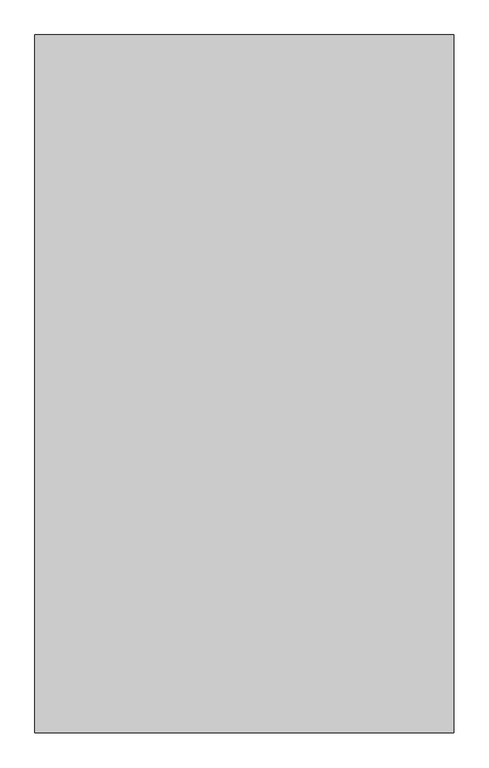
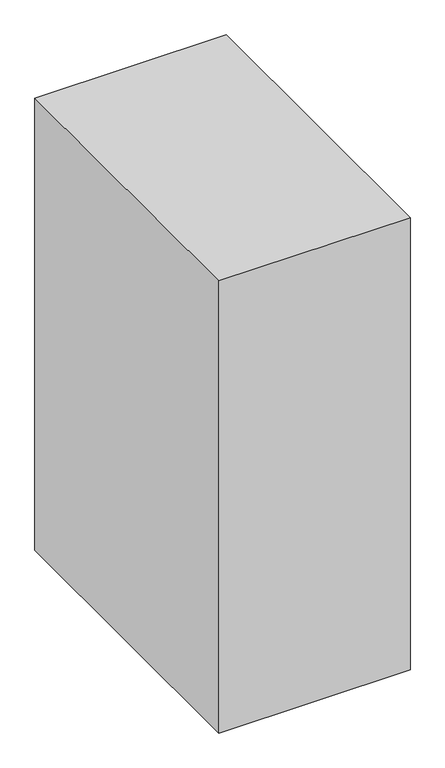
"""IFC4 building model written with IfcOpenShell, lengths in millimetres: proxy geometry, Space Planning Box_hec : Space Planning Box_hec."""

import ifcopenshell
import ifcopenshell.guid

model = None  # the IFC model being written
_history = None  # IfcOwnerHistory: only IFC2X3 demands one
_inside = {}  # id of a spatial element -> (the spatial element, [elements in it])
_under = {}  # id of a project, library or spatial element -> (it, [spatial elements below it])
_declared = {}  # id of a project -> (the project, [libraries it declares])
_typed = {}  # id of a type object -> (the type object, [elements of that type])
_made_of = {}  # id of a material, layer set ... -> (it, [elements and type objects made of it])


def new_model(schema):
    """Start an empty IFC model of exactly this schema.

    Asked for "IFC4X3", IfcOpenShell would pick the latest addendum, in which some entities
    have other attributes; the version numbers below select the first issue.
    IFC2X3 requires an IfcOwnerHistory on every rooted entity: one is made here for all.
    """
    global model, _history
    if schema == "IFC4X3":
        model = ifcopenshell.file(schema_version=(4, 3, 0, 0))
    else:
        model = ifcopenshell.file(schema=schema)
    _inside.clear()
    _under.clear()
    _declared.clear()
    _typed.clear()
    _made_of.clear()
    _history = None
    if model.schema == "IFC2X3":
        org = make("IfcOrganization", Name="unknown")
        user = make(
            "IfcPersonAndOrganization",
            ThePerson=make("IfcPerson", FamilyName="unknown"),
            TheOrganization=org,
        )
        app = make(
            "IfcApplication",
            ApplicationDeveloper=org,
            Version="unknown",
            ApplicationFullName="unknown",
            ApplicationIdentifier="unknown",
        )
        _history = make(
            "IfcOwnerHistory",
            OwningUser=user,
            OwningApplication=app,
            ChangeAction="ADDED",
            CreationDate=0,
        )
    return model


def make(cls, **values):
    """One entity of the class cls with the attributes given. An attribute that is None is left unset."""
    return model.create_entity(
        cls, **{name: value for name, value in values.items() if value is not None}
    )


def rooted(cls, **values):
    """An entity with a GlobalId (a new one), such as an element, a storey or a relation."""
    return make(cls, GlobalId=ifcopenshell.guid.new(), OwnerHistory=_history, **values)


def si_unit(unit_type, name, prefix=None):
    """IfcSIUnit, for example si_unit("LENGTHUNIT", "METRE", prefix="MILLI")."""
    return make("IfcSIUnit", UnitType=unit_type, Prefix=prefix, Name=name)


def assignment(units):
    """IfcUnitAssignment: the units of a project."""
    return None if units is None else make("IfcUnitAssignment", Units=units)


def point(xyz):
    """IfcCartesianPoint."""
    return None if xyz is None else make("IfcCartesianPoint", Coordinates=xyz)


def direction(xyz):
    """IfcDirection."""
    return None if xyz is None else make("IfcDirection", DirectionRatios=xyz)


def frame(location, z_axis=None, x_axis=None):
    """IfcAxis2Placement3D, a coordinate frame: its origin and axes. An axis left out is left unset."""
    return make(
        "IfcAxis2Placement3D",
        Location=point(location),
        Axis=direction(z_axis),
        RefDirection=direction(x_axis),
    )


def origin():
    """The frame at (0, 0, 0) with its axes left unset."""
    return frame((0.0, 0.0, 0.0))


def origin_with_axes():
    """The frame at (0, 0, 0) with the z axis (0, 0, 1) and the x axis (1, 0, 0) written out."""
    return frame((0.0, 0.0, 0.0), z_axis=(0.0, 0.0, 1.0), x_axis=(1.0, 0.0, 0.0))


def place(relative_to, where):
    """IfcLocalPlacement: puts the frame where relative to a parent placement (None: the world)."""
    return make(
        "IfcLocalPlacement", PlacementRelTo=relative_to, RelativePlacement=where
    )


def context(
    kind, dimensions, precision=None, world=None, true_north=None, identifier=None
):
    """IfcGeometricRepresentationContext, for example the 3D "Model" context."""
    return make(
        "IfcGeometricRepresentationContext",
        ContextIdentifier=identifier,
        ContextType=kind,
        CoordinateSpaceDimension=dimensions,
        Precision=precision,
        WorldCoordinateSystem=world,
        TrueNorth=true_north,
    )


def project(units=None, contexts=None):
    """IfcProject with its units and contexts."""
    return rooted(
        "IfcProject",
        Name="project",
        RepresentationContexts=contexts,
        UnitsInContext=assignment(units),
    )


def spatial(cls, under=None, at=None, **own):
    """A site, building, storey or space (cls), placed at a placement, below another one or the project."""
    s = rooted(cls, ObjectPlacement=at, **own)
    if under is not None:
        _under.setdefault(under.id(), (under, []))[1].append(s)
    return s


def polyline(points):
    """IfcPolyline through the points."""
    return make("IfcPolyline", Points=[point(p) for p in points])


def outline(outer, holes=None, kind="AREA"):
    """IfcArbitraryClosedProfileDef: a profile drawn as a closed curve; with holes, ...WithVoids."""
    if holes is None:
        return make("IfcArbitraryClosedProfileDef", ProfileType=kind, OuterCurve=outer)
    return make(
        "IfcArbitraryProfileDefWithVoids",
        ProfileType=kind,
        OuterCurve=outer,
        InnerCurves=holes,
    )


def extrude(swept, where, along, depth):
    """IfcExtrudedAreaSolid: the profile swept, set in the frame where, extruded along a direction by depth."""
    return make(
        "IfcExtrudedAreaSolid",
        SweptArea=swept,
        Position=where,
        ExtrudedDirection=direction(along),
        Depth=depth,
    )


def shape(context_of_items, identifier, shape_type, items):
    """IfcShapeRepresentation: the items that make up one representation, for example the "Body"."""
    return make(
        "IfcShapeRepresentation",
        ContextOfItems=context_of_items,
        RepresentationIdentifier=identifier,
        RepresentationType=shape_type,
        Items=items,
    )


def source(mapping_origin, context_of_items, identifier, shape_type, items):
    """IfcRepresentationMap: a shape defined once, which mapped items show again and again."""
    return make(
        "IfcRepresentationMap",
        MappingOrigin=mapping_origin,
        MappedRepresentation=shape(context_of_items, identifier, shape_type, items),
    )


def transform(
    local_origin,
    x_axis=None,
    y_axis=None,
    z_axis=None,
    scale=None,
    scale2=None,
    scale3=None,
    uniform=True,
):
    """IfcCartesianTransformationOperator3D, or its non-uniform kind. x_axis, y_axis, z_axis: its Axis1, 2, 3."""
    if uniform:
        return make(
            "IfcCartesianTransformationOperator3D",
            Axis1=direction(x_axis),
            Axis2=direction(y_axis),
            LocalOrigin=point(local_origin),
            Scale=scale,
            Axis3=direction(z_axis),
        )
    return make(
        "IfcCartesianTransformationOperator3DnonUniform",
        Axis1=direction(x_axis),
        Axis2=direction(y_axis),
        LocalOrigin=point(local_origin),
        Scale=scale,
        Axis3=direction(z_axis),
        Scale2=scale2,
        Scale3=scale3,
    )


def mapped(mapping_source, mapping_target):
    """IfcMappedItem: shows the shape of a source again, moved by a transform."""
    return make(
        "IfcMappedItem", MappingSource=mapping_source, MappingTarget=mapping_target
    )


def made_of(thing, what):
    """Note that an element or type object is made of a material, layer set ...; save() writes the relation."""
    if what is not None:
        _made_of.setdefault(what.id(), (what, []))[1].append(thing)
    return thing


def element(
    cls,
    number,
    at=None,
    inside=None,
    cuts=None,
    type_object=None,
    material=None,
    context=None,
    identifier="Body",
    shape_type=None,
    held_by="IfcProductDefinitionShape",
    body=None,
    shapes=None,
    **own,
):
    """One element of the class cls, such as IfcWall. Its Tag is "e" and its number.

    at: its placement. inside: the storey or other place that contains it. cuts: it is an
    opening in that element (IfcRelVoidsElement). A single representation is given by context,
    identifier, shape_type and body (its items); several are given by shapes. held_by: the class
    of the entity that holds the representations. save() writes the other relations.
    """
    e = rooted(cls, Tag="e%d" % number, ObjectPlacement=at, **own)
    if body is not None:
        shapes = [shape(context, identifier, shape_type, body)]
    if shapes is not None:
        e.Representation = make(held_by, Representations=shapes)
    if inside is not None:
        _inside.setdefault(inside.id(), (inside, []))[1].append(e)
    if cuts is not None:
        rooted(
            "IfcRelVoidsElement", RelatingBuildingElement=cuts, RelatedOpeningElement=e
        )
    if type_object is not None:
        _typed.setdefault(type_object.id(), (type_object, []))[1].append(e)
    return made_of(e, material)


def aggregate(whole, parts):
    """IfcRelAggregates: a whole, such as a stair, and the parts it consists of."""
    return rooted("IfcRelAggregates", RelatingObject=whole, RelatedObjects=parts)


def save(model, path):
    """Write the relations noted so far, then the file.

    IfcRelAggregates (storeys below a building ...), IfcRelContainedInSpatialStructure (elements
    in a storey), IfcRelDefinesByType, IfcRelAssociatesMaterial and IfcRelDeclares: one each for
    every whole, place, type object, material and project.
    """
    for whole, parts in _under.values():
        aggregate(whole, parts)
    for where, things in _inside.values():
        rooted(
            "IfcRelContainedInSpatialStructure",
            RelatedElements=things,
            RelatingStructure=where,
        )
    for kind, things in _typed.values():
        rooted("IfcRelDefinesByType", RelatedObjects=things, RelatingType=kind)
    for what, things in _made_of.values():
        rooted("IfcRelAssociatesMaterial", RelatedObjects=things, RelatingMaterial=what)
    for by, libraries in _declared.values():
        rooted("IfcRelDeclares", RelatingContext=by, RelatedDefinitions=libraries)
    model.write(path)


def generic_models_47b98be1(model_context):
    return source(origin(), model_context, "Body", "SweptSolid", [
        extrude(outline(polyline([(1200.0, 2000.0), (1200.0, -2000.0), (-1200.0, -2000.0), (-1200.0, 2000.0), (1200.0, 2000.0)])), origin_with_axes(), (0.0, 0.0, 1.0), 6000.0),
    ])


if __name__ == "__main__":
    model = new_model("IFC4")
    model_context = context("Model", 3, world=origin())
    ifc_project = project(units=[si_unit("LENGTHUNIT", "METRE", prefix="MILLI")], contexts=[model_context])
    site = spatial("IfcSite", under=ifc_project)
    building = spatial("IfcBuilding", under=site)
    placement = place(None, origin())
    generic_models_shape = generic_models_47b98be1(model_context)
    element("IfcBuildingElementProxy", 1, Name="Space Planning Box_hec : Space Planning Box_hec", ObjectType="Space Planning Box_hec : Space Planning Box_hec", at=placement, inside=building, context=model_context, shape_type="MappedRepresentation", body=[
        mapped(generic_models_shape, transform((0.0, 0.0, 0.0), x_axis=(1.0, 0.0, 0.0), y_axis=(0.0, 1.0, 0.0), z_axis=(0.0, 0.0, 1.0))),
    ])
    save(model, "model.ifc")

# Revit data of these elements
# Type "Space Planning Box_hec : Space Planning Box_hec"
#   Type Comments = "..."
#   Room Name [instance default] = "?"
#   Interior Finish [instance default] = ""
#   Exterior Finish [instance default] = ""
#   Department [instance default] = ""
#   Assembly Code = "..."
#   Width [instance default] = 1524 mm
#   Program Area [instance default] = 0 m²
#   Length [instance default] = 1524 mm
#   Height [instance default] = 1524 mm
#   Area [instance default] = 2.32258 m²
#   Fill Color [instance default] = Cyan
#   Default Elevation = 0
# Element 1 (IfcBuildingElementProxy, "Space Planning Box_hec : Space Planning Box_hec")
#   Room Name = "Locker Room (F)"
#   Interior Finish = "IF2-1"
#   Exterior Finish = "EF1"
#   Department = "AR"
#   Width = 2400 mm
#   Program Area = 31.5 m²
#   Length = 4000 mm
#   Height = 6000 mm
#   Area = 9.6 m²
#   Fill Color = Lavender
#   Materials on its faces: "Lavender"
# Materials
#   "Cyan": class "Generic", colour RGB 0 255 255, transparency 0.2, Cost = 0
#   "Lavender": class "Generic", colour RGB 186 85 211, transparency 0.2, Cost = 0
